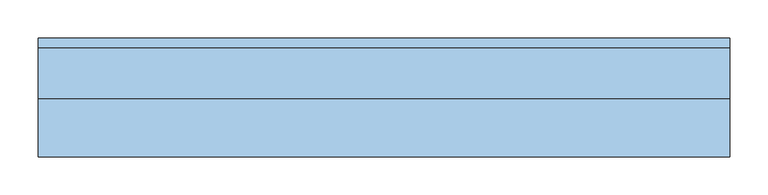
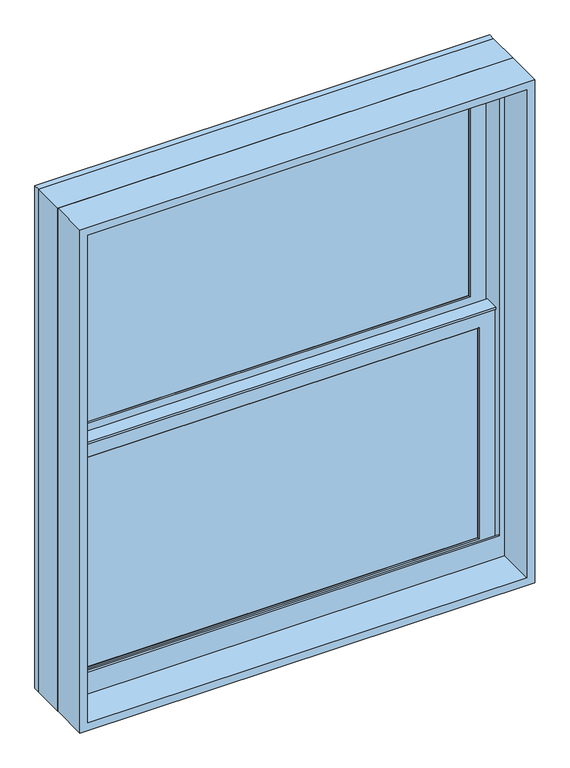
"""IFC4 building model written with IfcOpenShell, lengths in millimetres: window geometry, Window-Double_Hung-Marvin-Essential : ESDH3036."""

from ifc_helpers import new_model, si_unit, frame, origin, place, context, project, spatial, polyline, outline, extrude, faceted_brep, source, transform, mapped, element, save


def window_a6eb63ae(model_context):
    return source(origin(), model_context, "Body", "SolidModel", [
        extrude(outline(polyline([(140.7583333, 20.6375), (140.7583333, 15.875), (121.7083333, 15.875), (121.7083333, 20.6375), (140.7583333, 20.6375)])), frame((0.0, 0.0, 1441.45), z_axis=(0.0, 0.0, 1.0), x_axis=(1.0, 0.0, 0.0)), (0.0, 0.0, 1.0), 450.85),
        extrude(outline(polyline([(-121.7083333, 20.6375), (-121.7083333, 15.875), (-140.7583333, 15.875), (-140.7583333, 20.6375), (-121.7083333, 20.6375)])), frame((0.0, 0.0, 1441.45), z_axis=(0.0, 0.0, 1.0), x_axis=(1.0, 0.0, 0.0)), (0.0, 0.0, 1.0), 450.85),
        extrude(outline(polyline([(393.7, 20.6375), (393.7, 15.875), (-393.7, 15.875), (-393.7, 20.6375), (393.7, 20.6375)])), frame((0.0, 0.0, 1657.35), z_axis=(0.0, 0.0, 1.0), x_axis=(1.0, 0.0, 0.0)), (0.0, 0.0, 1.0), 19.05),
        extrude(outline(polyline([(-140.7583333, 46.83125), (-140.7583333, 51.59375), (-121.7083333, 51.59375), (-121.7083333, 46.83125), (-140.7583333, 46.83125)])), frame((0.0, 0.0, 1930.4), z_axis=(0.0, 0.0, 1.0), x_axis=(1.0, 0.0, 0.0)), (0.0, 0.0, 1.0), 450.85),
        extrude(outline(polyline([(121.7083333, 46.83125), (121.7083333, 51.59375), (140.7583333, 51.59375), (140.7583333, 46.83125), (121.7083333, 46.83125)])), frame((0.0, 0.0, 1930.4), z_axis=(0.0, 0.0, 1.0), x_axis=(1.0, 0.0, 0.0)), (0.0, 0.0, 1.0), 450.85),
        extrude(outline(polyline([(-393.7, 46.83125), (-393.7, 51.59375), (393.7, 51.59375), (393.7, 46.83125), (-393.7, 46.83125)])), frame((0.0, 0.0, 2146.3), z_axis=(0.0, 0.0, 1.0), x_axis=(1.0, 0.0, 0.0)), (0.0, 0.0, 1.0), 19.05),
        extrude(outline(polyline([(140.7583333, 20.6375), (121.7083333, 20.6375), (121.7083333, 25.4), (140.7583333, 25.4), (140.7583333, 20.6375)])), frame((0.0, 0.0, 1441.45), z_axis=(0.0, 0.0, 1.0), x_axis=(1.0, 0.0, 0.0)), (0.0, 0.0, 1.0), 450.85),
        extrude(outline(polyline([(-121.7083333, 20.6375), (-140.7583333, 20.6375), (-140.7583333, 25.4), (-121.7083333, 25.4), (-121.7083333, 20.6375)])), frame((0.0, 0.0, 1441.45), z_axis=(0.0, 0.0, 1.0), x_axis=(1.0, 0.0, 0.0)), (0.0, 0.0, 1.0), 450.85),
        extrude(outline(polyline([(393.7, 20.6375), (-393.7, 20.6375), (-393.7, 25.4), (393.7, 25.4), (393.7, 20.6375)])), frame((0.0, 0.0, 1657.35), z_axis=(0.0, 0.0, 1.0), x_axis=(1.0, 0.0, 0.0)), (0.0, 0.0, 1.0), 19.05),
        extrude(outline(polyline([(-140.7583333, 56.35625), (-121.7083333, 56.35625), (-121.7083333, 51.59375), (-140.7583333, 51.59375), (-140.7583333, 56.35625)])), frame((0.0, 0.0, 1930.4), z_axis=(0.0, 0.0, 1.0), x_axis=(1.0, 0.0, 0.0)), (0.0, 0.0, 1.0), 450.85),
        extrude(outline(polyline([(121.7083333, 56.35625), (140.7583333, 56.35625), (140.7583333, 51.59375), (121.7083333, 51.59375), (121.7083333, 56.35625)])), frame((0.0, 0.0, 1930.4), z_axis=(0.0, 0.0, 1.0), x_axis=(1.0, 0.0, 0.0)), (0.0, 0.0, 1.0), 450.85),
        extrude(outline(polyline([(-393.7, 56.35625), (393.7, 56.35625), (393.7, 51.59375), (-393.7, 51.59375), (-393.7, 56.35625)])), frame((0.0, 0.0, 2146.3), z_axis=(0.0, 0.0, 1.0), x_axis=(1.0, 0.0, 0.0)), (0.0, 0.0, 1.0), 19.05),
        faceted_brep([(-420.6875, 5.6780605, 1922.3351748), (-420.6875, 5.6780605, 1917.7), (420.6875, 5.6780605, 1917.7), (420.6875, 5.6780605, 1922.3351748), (-420.6875, 34.8118605, 1922.3351748), (420.6875, 34.8118605, 1922.3351748), (420.6875, 34.8118605, 1917.7), (-420.6875, 34.8118605, 1917.7), (-420.6875, 30.1625, 1917.7), (-420.6875, 30.1625, 1414.4625), (-420.6875, 8.9241104, 1414.4625), (-420.6875, 8.9241104, 1917.7), (420.6875, 8.9241104, 1917.7), (420.6875, 30.1625, 1917.7), (420.6875, 8.9241104, 1414.4625), (420.6875, 30.1625, 1414.4625), (-404.8034752, 11.90625, 1903.4034752), (-404.8034752, 30.1625, 1903.4034752), (404.8034752, 30.1625, 1903.4034752), (404.8034752, 11.90625, 1903.4034752), (-388.14375, 10.4662439, 1886.74375), (-388.14375, 11.90625, 1886.74375), (388.14375, 11.90625, 1886.74375), (388.14375, 10.4662439, 1886.74375), (389.6858834, 8.9241104, 1888.2858834), (-389.6858834, 8.9241104, 1888.2858834), (404.8034752, 30.1625, 1430.3465248), (404.8034752, 11.90625, 1430.3465248), (388.14375, 11.90625, 1447.00625), (388.14375, 10.4662439, 1447.00625), (389.6858834, 8.9241104, 1445.4641166), (-404.8034752, 30.1625, 1430.3465248), (-404.8034752, 11.90625, 1430.3465248), (-388.14375, 11.90625, 1447.00625), (-388.14375, 10.4662439, 1447.00625), (-389.6858834, 8.9241104, 1445.4641166)], [[[0, 1, 2, 3]], [[4, 5, 6, 7]], [[1, 0, 4, 7, 8, 9, 10, 11]], [[2, 1, 11, 12]], [[7, 6, 13, 8]], [[3, 2, 12, 14, 15, 13, 6, 5]], [[0, 3, 5, 4]], [[16, 17, 18, 19]], [[20, 21, 22, 23]], [[20, 23, 24, 25]], [[19, 18, 26, 27]], [[23, 22, 28, 29]], [[24, 23, 29, 30]], [[27, 26, 31, 32]], [[29, 28, 33, 34]], [[30, 29, 34, 35]], [[15, 14, 10, 9]], [[15, 9, 8, 13], [18, 17, 31, 26]], [[17, 16, 32, 31]], [[16, 19, 27, 32], [22, 21, 33, 28]], [[21, 20, 34, 33]], [[20, 25, 35, 34]], [[10, 14, 12, 11], [25, 24, 30, 35]]]),
        extrude(outline(polyline([(38.5955581, 1903.4125), (33.5778968, 1903.4125), (33.5778968, 1905.0), (39.9405976, 1905.0), (39.9405976, 1903.4125), (61.515625, 1903.4125), (47.6307501, 1900.0975159), (38.5955581, 1900.0975159), (38.5955581, 1903.4125)])), frame((-420.6875, 0.0, 0.0), z_axis=(1.0, 0.0, 0.0), x_axis=(0.0, 1.0, 0.0)), (0.0, 0.0, 1.0), 841.375),
        faceted_brep([(450.85, 0.0, 1384.3), (450.85, 0.0, 2438.4), (-450.85, 0.0, 2438.4), (-450.85, 0.0, 1384.3), (424.65625, 0.0, 1445.41875), (-424.65625, 0.0, 1445.41875), (-424.65625, 0.0, 2412.20625), (424.65625, 0.0, 2412.20625), (424.65625, 3.96875, 1384.3), (-424.65625, 3.96875, 1384.3), (-424.65625, 3.96875, 1445.41875), (424.65625, 3.96875, 1445.41875), (-450.85, 65.6828125, 1384.3), (-424.65625, 65.6828125, 1384.3), (424.65625, 65.6828125, 1384.3), (450.85, 65.6828125, 1384.3), (-450.85, 65.6828125, 2438.4), (450.85, 65.6828125, 2438.4), (424.65625, 65.6828125, 2412.20625), (-424.65625, 65.6828125, 2412.20625)], [[[0, 1, 2, 3], [4, 5, 6, 7]], [[8, 9, 10, 11]], [[5, 4, 11, 10]], [[0, 3, 12, 13, 9, 8, 14, 15]], [[13, 12, 16, 17, 15, 14, 18, 19]], [[13, 19, 6, 5, 10, 9]], [[7, 6, 19, 18]], [[18, 14, 8, 11, 4, 7]], [[1, 0, 15, 17]], [[2, 1, 17, 16]], [[3, 2, 16, 12]]]),
        faceted_brep([(424.65625, 30.1625, 1911.35), (423.06875, 30.1625, 1911.35), (423.06875, 30.1625, 1408.6544613), (424.65625, 30.1625, 1408.6544613), (-423.06875, 30.1625, 1911.35), (-424.65625, 30.1625, 1911.35), (-424.65625, 30.1625, 1408.6544613), (-423.06875, 30.1625, 1408.6544613), (423.06875, 63.5, 1911.35), (424.65625, 63.5, 1911.35), (424.65625, 63.5, 1402.1743077), (423.06875, 63.5, 1402.1743077), (-424.65625, 63.5, 1911.35), (-423.06875, 63.5, 1911.35), (-423.06875, 63.5, 1402.1743077), (-424.65625, 63.5, 1402.1743077), (435.9108932, 3.96875, 1413.7460105), (435.9108932, 3.96875, 1384.3), (435.9108932, 65.6828125, 1384.3), (435.9108932, 65.6828125, 1401.750012), (-435.9108932, 3.96875, 1384.3), (-435.9108932, 3.96875, 1413.7460105), (-435.9108932, 65.6828125, 1401.750012), (-435.9108932, 65.6828125, 1384.3), (435.9108932, 78.58125, 1399.2428097), (-435.9108932, 78.58125, 1399.2428097), (-433.8971252, 68.2348864, 1401.2539391), (-415.93135, 68.2348864, 1401.2539391), (-415.93135, 65.6828125, 1401.750012), (415.93135, 65.6828125, 1401.750012), (415.93135, 68.2348864, 1401.2539391), (433.8971252, 68.2348864, 1401.2539391), (-450.85, 65.6828125, 1384.3), (-450.85, 78.5948249, 1384.3), (450.85, 78.5948249, 1384.3), (450.85, 65.6828125, 1384.3), (-450.85, 78.58125, 2438.4), (450.85, 78.58125, 2438.4), (435.9108932, 78.58125, 2423.4608932), (-435.9108932, 78.58125, 2423.4608932), (-450.85, 65.6828125, 2438.4), (-433.8971252, 68.2348864, 2421.4471252), (433.8971252, 68.2348864, 2421.4471252), (415.93135, 68.2348864, 2403.48135), (-415.93135, 68.2348864, 2403.48135), (-415.93135, 65.6828125, 2403.48135), (415.93135, 65.6828125, 2403.48135), (450.85, 65.6828125, 2438.4)], [[[0, 1, 2, 3]], [[4, 5, 6, 7]], [[8, 9, 10, 11]], [[12, 13, 14, 15]], [[1, 8, 11, 2]], [[9, 0, 3, 10]], [[1, 0, 9, 8]], [[5, 4, 13, 12]], [[5, 12, 15, 6]], [[13, 4, 7, 14]], [[16, 17, 18, 19]], [[20, 21, 22, 23]], [[24, 25, 26, 27, 28, 22, 21, 16, 19, 29, 30, 31], [3, 2, 11, 10], [7, 6, 15, 14]], [[17, 16, 21, 20]], [[17, 20, 23, 32, 33, 34, 35, 18]], [[34, 33, 36, 37], [25, 24, 38, 39]], [[33, 32, 40, 36]], [[39, 41, 26, 25]], [[41, 42, 31, 30, 43, 44, 27, 26]], [[44, 45, 28, 27]], [[40, 32, 23, 22, 28, 45, 46, 29, 19, 18, 35, 47]], [[36, 40, 47, 37]], [[39, 38, 42, 41]], [[44, 43, 46, 45]], [[34, 37, 47, 35]], [[42, 38, 24, 31]], [[46, 43, 30, 29]]]),
        extrude(outline(polyline([(400.84375, 11.90625), (-400.84375, 11.90625), (-400.84375, 15.08125), (400.84375, 15.08125), (400.84375, 11.90625)])), frame((0.0, 0.0, 1434.30625), z_axis=(0.0, 0.0, 1.0), x_axis=(1.0, 0.0, 0.0)), (0.0, 0.0, 1.0), 465.1375),
        extrude(outline(polyline([(400.84375, 42.8625), (-400.84375, 42.8625), (-400.84375, 46.0375), (400.84375, 46.0375), (400.84375, 42.8625)])), frame((0.0, 0.0, 1923.25625), z_axis=(0.0, 0.0, 1.0), x_axis=(1.0, 0.0, 0.0)), (0.0, 0.0, 1.0), 465.1375),
        faceted_brep([(-388.14375, 31.194477, 1886.74375), (-389.6858834, 32.7366104, 1888.2858834), (389.6858834, 32.7366104, 1888.2858834), (388.14375, 31.194477, 1886.74375), (-388.14375, 30.1625, 1886.74375), (388.14375, 30.1625, 1886.74375), (-420.6875, 32.7366104, 1919.2875), (-420.6875, 30.1625, 1919.2875), (420.6875, 30.1625, 1919.2875), (420.6875, 32.7366104, 1919.2875), (389.6858834, 32.7366104, 1445.4641166), (388.14375, 31.194477, 1447.00625), (388.14375, 30.1625, 1447.00625), (420.6875, 30.1625, 1414.4625), (420.6875, 32.7366104, 1414.4625), (-389.6858834, 32.7366104, 1445.4641166), (-388.14375, 31.194477, 1447.00625), (-388.14375, 30.1625, 1447.00625), (-420.6875, 30.1625, 1414.4625), (-420.6875, 32.7366104, 1414.4625)], [[[0, 1, 2, 3]], [[4, 0, 3, 5]], [[6, 7, 8, 9]], [[3, 2, 10, 11]], [[5, 3, 11, 12]], [[9, 8, 13, 14]], [[11, 10, 15, 16]], [[12, 11, 16, 17]], [[14, 13, 18, 19]], [[9, 14, 19, 6], [1, 15, 10, 2]], [[16, 15, 1, 0]], [[17, 16, 0, 4]], [[7, 18, 13, 8], [5, 12, 17, 4]], [[19, 18, 7, 6]]]),
        faceted_brep([(-404.8034752, 42.8625, 2392.3534752), (-404.8034752, 61.11875, 2392.3534752), (404.8034752, 61.11875, 2392.3534752), (404.8034752, 42.8625, 2392.3534752), (-388.14375, 41.4224939, 2375.69375), (-388.14375, 42.8625, 2375.69375), (388.14375, 42.8625, 2375.69375), (388.14375, 41.4224939, 2375.69375), (-389.6858834, 39.8803604, 2377.2358834), (389.6858834, 39.8803604, 2377.2358834), (-420.6875, 61.11875, 2408.2375), (-420.6875, 39.8803604, 2408.2375), (420.6875, 39.8803604, 2408.2375), (420.6875, 61.11875, 2408.2375), (404.8034752, 61.11875, 1919.2965248), (404.8034752, 42.8625, 1919.2965248), (388.14375, 42.8625, 1935.95625), (388.14375, 41.4224939, 1935.95625), (389.6858834, 39.8803604, 1934.4141166), (420.6875, 39.8803604, 1903.4125), (420.6875, 61.11875, 1903.4125), (-404.8034752, 61.11875, 1919.2965248), (-404.8034752, 42.8625, 1919.2965248), (-388.14375, 42.8625, 1935.95625), (-388.14375, 41.4224939, 1935.95625), (-389.6858834, 39.8803604, 1934.4141166), (-420.6875, 39.8803604, 1903.4125), (-420.6875, 61.11875, 1903.4125)], [[[0, 1, 2, 3]], [[4, 5, 6, 7]], [[8, 4, 7, 9]], [[10, 11, 12, 13]], [[3, 2, 14, 15]], [[7, 6, 16, 17]], [[9, 7, 17, 18]], [[13, 12, 19, 20]], [[15, 14, 21, 22]], [[17, 16, 23, 24]], [[18, 17, 24, 25]], [[20, 19, 26, 27]], [[13, 20, 27, 10], [1, 21, 14, 2]], [[22, 21, 1, 0]], [[3, 15, 22, 0], [5, 23, 16, 6]], [[24, 23, 5, 4]], [[25, 24, 4, 8]], [[11, 26, 19, 12], [9, 18, 25, 8]], [[27, 26, 11, 10]]]),
        faceted_brep([(-420.6875, 61.11875, 1903.4125), (-420.6875, 63.6928604, 1903.4125), (420.6875, 63.6928604, 1903.4125), (420.6875, 61.11875, 1903.4125), (-388.14375, 62.150727, 1935.95625), (-388.14375, 61.11875, 1935.95625), (388.14375, 61.11875, 1935.95625), (388.14375, 62.150727, 1935.95625), (-389.6858834, 63.6928604, 1934.4141166), (389.6858834, 63.6928604, 1934.4141166), (420.6875, 63.6928604, 2408.2375), (420.6875, 61.11875, 2408.2375), (388.14375, 61.11875, 2375.69375), (388.14375, 62.150727, 2375.69375), (389.6858834, 63.6928604, 2377.2358834), (-420.6875, 63.6928604, 2408.2375), (-420.6875, 61.11875, 2408.2375), (-388.14375, 61.11875, 2375.69375), (-388.14375, 62.150727, 2375.69375), (-389.6858834, 63.6928604, 2377.2358834)], [[[0, 1, 2, 3]], [[4, 5, 6, 7]], [[8, 4, 7, 9]], [[3, 2, 10, 11]], [[7, 6, 12, 13]], [[9, 7, 13, 14]], [[11, 10, 15, 16]], [[13, 12, 17, 18]], [[14, 13, 18, 19]], [[16, 15, 1, 0]], [[3, 11, 16, 0], [5, 17, 12, 6]], [[18, 17, 5, 4]], [[19, 18, 4, 8]], [[1, 15, 10, 2], [9, 14, 19, 8]]]),
        extrude(outline(polyline([(400.84375, 26.19375), (-400.84375, 26.19375), (-400.84375, 30.1625), (400.84375, 30.1625), (400.84375, 26.19375)])), frame((0.0, 0.0, 1434.30625), z_axis=(0.0, 0.0, 1.0), x_axis=(1.0, 0.0, 0.0)), (0.0, 0.0, 1.0), 465.1375),
        extrude(outline(polyline([(400.84375, 57.15), (-400.84375, 57.15), (-400.84375, 61.11875), (400.84375, 61.11875), (400.84375, 57.15)])), frame((0.0, 0.0, 1923.25625), z_axis=(0.0, 0.0, 1.0), x_axis=(1.0, 0.0, 0.0)), (0.0, 0.0, 1.0), 465.1375),
        extrude(outline(polyline([(2438.4, 450.85), (2438.4, -450.85), (1384.3, -450.85), (1384.3, 450.85), (2438.4, 450.85)]), holes=[polyline([(2422.525, 434.975), (1400.175, 434.975), (1400.175, -434.975), (2422.525, -434.975), (2422.525, 434.975)])]), frame((0.0, -76.2, 0.0), z_axis=(0.0, 1.0, 0.0), x_axis=(0.0, 0.0, 1.0)), (0.0, 0.0, 1.0), 75.40625),
    ])


if __name__ == "__main__":
    model = new_model("IFC4")
    model_context = context("Model", 3, world=origin())
    ifc_project = project(units=[si_unit("LENGTHUNIT", "METRE", prefix="MILLI")], contexts=[model_context])
    site = spatial("IfcSite", under=ifc_project)
    building = spatial("IfcBuilding", under=site)
    placement = place(None, origin())
    window_shape = window_a6eb63ae(model_context)
    element("IfcWindow", 1, ObjectType="Window-Double_Hung-Marvin-Essential : ESDH3036", at=placement, inside=building, context=model_context, shape_type="MappedRepresentation", body=[
        mapped(window_shape, transform((0.0, 0.0, 0.0), x_axis=(1.0, 0.0, 0.0), y_axis=(0.0, 1.0, 0.0), z_axis=(0.0, 0.0, 1.0))),
    ])
    save(model, "model.ifc")

# Revit data of these elements
# Type "Window-Double_Hung-Marvin-Essential : ESDH3036"
#   Type Mark = "44"
#   Window Type = "Essential Double Hung"
#   Product data url = "https://bimobject.com/marvin-windows-and-doors/product/marvin-dhwau"
#   Product Guid = "c4a96547-874c-4385-91dc-a058adc19d98"
#   Frame = "All Ultrex"
#   Egress Window = "No"
#   URL = "www.marvin.com"
#   Model = "ESDH3036"
#   Manufacturer = "Marvin Windows and Doors"
#   Label Egress = ""
#   Glass Type = "IG Low E II with Argon"
#   Design Pressure = "DP50"
#   Description = "3642 DBHG"
#   Analytic Construction = "<None>"
#   Prairie Corner Width = 0' - 4"
#   Prairie Corner Height = 0' - 4"
#   Egress Width = 2' - 8 9/16"
#   Egress Height = 1' - 4 27/128"
#   Rough Width = 3' - 0"
#   Rough Height = 3' - 6"
#   Nominal Width = 3' - 0"
#   Nominal Height = 3' - 6"
#   Inset to Installation Flange [instance default] = 0' - 1"
#   Height = 3' - 5 1/2"
#   Egress Area = 3.66575 SF
#   Default Head Height = 8' - 0"
#   Width = 2' - 11 1/2"
#   Daylight Area = 7.3488 SF
#   DLO Width = 2' - 6 9/16"
#   DLO Height = 1' - 5 5/16"
#   Muntins Top Sash = yes
#   Lites Wide Top Sash = 3
#   Lites Wide Bottom Sash = 3
#   Lites High Top Sash = 2
#   Lites High Bottom Sash = 2
#   Lite Cut Prairie 9 = no
#   Lite Cut HV Grid = yes
#   Muntins Bottom Sash = yes
#   Label Visibility = no
#   Jamb Extension Visibility = yes
#   Edition number = 1
#   Interior Material = Ultrex-Marvin-Stonewhite
#   Glazing Material = Glass-Marvin-IG Low E II with Argon
#   Cladding Material = Ultrex-Marvin-Pebblegray
#   Wall Closure = (empty or 0)
#   Assembly Code = ""
# Element 1 (IfcWindow, "Window-Double_Hung-Marvin-Essential : ESDH3036")
#   Materials on its faces: "Ultrex-Marvin-Pebblegray", "Ultrex-Marvin-Stonewhite", "Glass-Marvin-IG Low E II with Argon"
# Materials
#   "Ultrex-Marvin-Stonewhite": class "Paint", colour RGB 250 251 245, transparency 0
#   "Glass-Marvin-IG Low E II with Argon": class "Glass", colour RGB 0 128 192, transparency 0.85
#   "Ultrex-Marvin-Pebblegray": class "Paint", colour RGB 189 185 173, transparency 0
